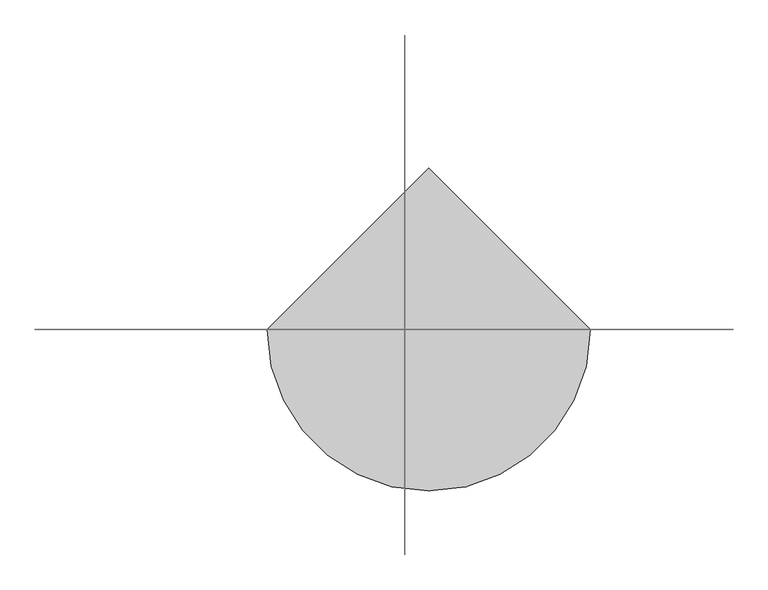
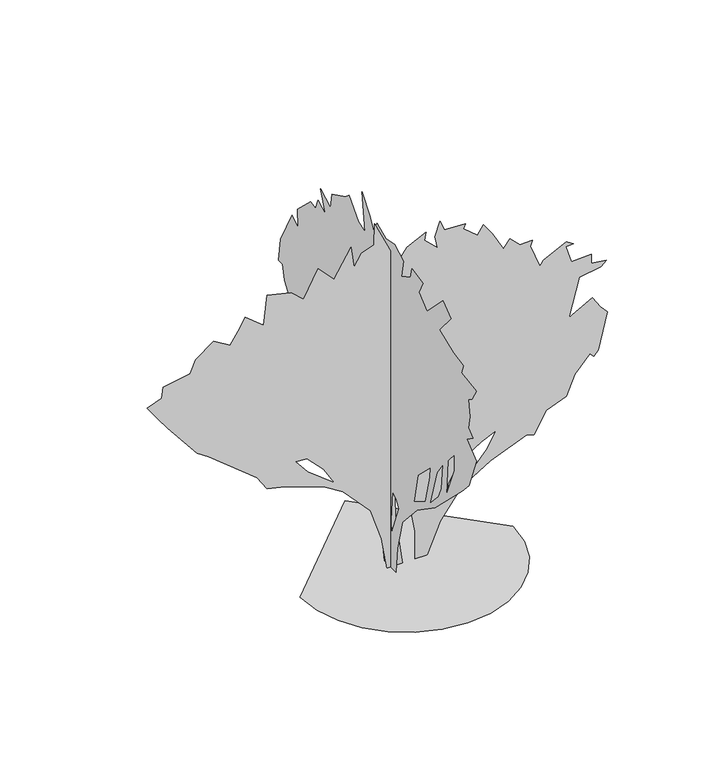
"""IFC4 building model written with IfcOpenShell, lengths in millimetres: proxy geometry, honey myrtle 26117 : honey myrtle 26117."""

from ifc_helpers import new_model, si_unit, origin, place, context, project, spatial, triangles, source, transform, mapped, element, save


def entourage_6475341c(model_context):
    return source(origin(), model_context, "Body", "Tessellation", [
        triangles([(-396.3767504, 0.0, 8.22e-05), (-385.8992649, -90.8237077, 8.22e-05), (-356.0543206, -174.2306261, 8.22e-05), (-309.2370838, -247.8313661, 8.22e-05), (-247.8313661, -309.2370838, 8.22e-05), (-174.2306261, -356.0543206, 8.22e-05), (-90.8237077, -385.8992649, 8.22e-05), (1.73e-05, -396.3767504, 8.22e-05), (90.8237077, -385.8992649, 8.22e-05), (174.2306261, -356.0543206, 8.22e-05), (247.8313661, -309.2370838, 8.22e-05), (309.2370838, -247.8313661, 8.22e-05), (356.0543206, -174.2306261, 8.22e-05), (385.8992649, -90.8237077, 8.22e-05), (396.3767504, 3.47e-05, 8.22e-05), (-5.2e-05, 396.3767504, 8.22e-05), (-59.3577095, -35.0059915, 9.26e-05), (-59.3577095, -44.8705806, 101.5460546), (-59.3577095, -75.4742449, 222.0478563), (-59.3577095, -168.9964434, 326.3007588), (-59.3577095, -285.8741748, 405.6706235), (-59.3579639, -459.2340692, 576.3228888), (-59.3579639, -503.9253456, 625.6344137), (-59.3579639, -553.1479589, 751.1941189), (-59.3579639, -491.6190474, 799.7715317), (-59.3579639, -530.478485, 828.915465), (-59.3579639, -501.3320083, 851.5849388), (-59.3579639, -511.0474763, 900.1598808), (-59.3579639, -501.3320083, 961.688756), (-59.3579639, -524.0014821, 977.8812269), (-59.3579639, -553.1479589, 1026.4561689), (-59.3579639, -455.9955677, 1039.4101748), (-59.3579639, -469.4956884, 1077.0376745), (-59.3579639, -404.1821606, 1087.9850441), (-59.3579639, -313.5068087, 1123.6085238), (-59.3579639, -387.9896896, 1211.0454105), (-59.3579639, -336.1762825, 1249.9048119), (-59.3579639, -235.7859349, 1149.5164627), (-59.3579639, -183.9712561, 1191.6144018), (-59.3579639, -209.8784683, 1243.4278816), (-59.3579639, -138.9198272, 1256.3183739), (-59.3579639, -128.9188388, 1217.5224134), (-59.3579639, -70.6279291, 1185.1373989), (-59.3579639, -83.5816624, 1253.143277), (-59.3579639, -25.4436618, 1284.1769932), (-59.3579639, 29.761912, 1272.5743584), (-59.3579639, 86.0073592, 1299.3586246), (-59.3579639, 110.7212849, 1256.3817421), (-59.3579639, 133.3899957, 1298.4822247), (-59.3579639, 185.2039207, 1363.2496376), (-59.3577095, 165.7739475, 1217.5224134), (-59.3577095, 207.8728858, 1230.4738758), (-59.3577095, 266.3644464, 1299.9199276), (-59.3577095, 292.0717617, 1279.0512886), (-59.3577095, 376.2676217, 1236.950806), (-59.3577095, 385.9830897, 1178.660396), (-59.3577095, 450.7505027, 1214.2838757), (-59.3577095, 418.3680679, 1133.3239918), (-59.3577095, 466.9429736, 1159.22946), (-59.3577095, 484.2835213, 1117.1086298), (-59.3577095, 515.5204227, 1123.6085238), (-59.3577095, 599.7162646, 1042.6486399), (-59.3577095, 596.4777632, 974.6427618), (-59.3577095, 635.3397079, 997.3122356), (-59.3577095, 709.8225889, 858.0619417), (-59.3577095, 722.7765947, 767.3865898), (-59.3577095, 696.8686558, 767.3865898), (-59.3577095, 683.91465, 712.3346449), (-59.3577095, 619.147237, 621.659293), (-59.3577095, 586.7622588, 628.1362959), (-59.3577095, 577.0493342, 595.7513177), (-59.3577095, 544.664356, 589.2743148), (-59.3577095, 512.2819213, 514.7914338), (-59.3577095, 453.9890041, 501.8400078), (-59.3577095, 473.4199765, 479.1705339), (-59.3577095, 438.083507, 433.2245012), (-59.3577095, 424.8450708, 430.5955919), (-59.3577095, 359.671251, 388.3935531), (-59.3577095, 230.5626891, 332.9860339), (-59.3577095, 112.6590482, 224.7923109), (-59.3577095, 55.1474106, 87.2636415), (-59.3577095, 39.476642, 8.38e-05), (-59.3577095, -5.8605105, 135.9018064), (-59.3577095, -2.7896791, 186.1833303), (-59.3577095, -12.337225, 304.2967785), (-59.3577095, -38.2442317, 288.1068329), (-59.3577095, -54.4362076, 262.1988576), (-59.3577095, -151.5875587, 349.6357444), (-59.3577095, -177.4947618, 469.4550296), (-59.3577095, -258.4549001, 547.176412), (-59.3577095, -255.2163986, 508.3169744), (-59.3577095, -226.0704487, 394.9721486), (-59.3577095, -255.2163986, 404.687653), (-59.3577095, -297.3143196, 550.4149135), (-59.3577095, -337.517407, 606.5056758), (-59.3577095, -326.4607781, 505.0785092), (-59.3577095, -307.0298058, 462.9780267), (-59.3577095, -358.8432129, 501.8400078), (-59.3579639, -368.5587173, 641.0903017), (-59.3579639, -410.6591635, 689.6651711), (-59.3579639, -410.6591635, 628.1362959), (-59.3577095, 198.157654, 356.112711), (-59.3577095, 261.769596, 391.7057055), (-59.3577095, 324.4541782, 475.9320325), (-59.3577095, 282.3562755, 469.4550296), (-59.3577095, 253.2100531, 430.5955919), (-267.2940953, 2.61e-05, 404.687653), (-308.6096875, 2.21e-05, 471.3142911), (-370.9208914, 1.84e-05, 534.2224425), (-413.0213739, 1.82e-05, 537.4609076), (-368.4215527, 2.15e-05, 482.1804156), (30.6369404, 5.02e-05, 0.0), (31.1304627, 4.38e-05, 108.1619844), (9.0696959, 3.61e-05, 237.4841779), (-47.0839311, 3.05e-05, 330.2047357), (-39.4309189, 4.01e-05, 170.4041154), (-14.7000316, 5.02e-05, 0.0), (-72.990889, 5.02e-05, 0.0), (-92.9872747, 4.29e-05, 122.5858678), (-134.4006626, 3.55e-05, 247.1552083), (-236.0793036, 2.88e-05, 358.7517941), (-302.2063538, 2.64e-05, 398.8659516), (-451.8807753, 2.32e-05, 453.2625587), (-519.8892331, 2.22e-05, 469.4550296), (-555.510133, 1.89e-05, 524.5069382), (-736.858366, 1.03e-05, 670.234235), (-778.9587759, 8.5e-06, 699.3807117), (-889.0625931, 4e-07, 835.3924679), (-924.6860727, -2.5e-06, 883.9674099), (-965.6003632, -6e-06, 942.4685629), (-911.7320669, -7.1e-06, 961.688756), (-905.255064, -9.6e-06, 1003.7892385), (-804.8642441, -1.06e-05, 1019.979166), (-785.4357788, -1.35e-05, 1068.5565788), (-717.4299007, -1.64e-05, 1117.1315208), (-655.8984821, -1.43e-05, 1081.5105846), (-620.2775459, -1.75e-05, 1136.5625296), (-600.8465735, -1.97e-05, 1172.1833931), (-532.8406591, -1.64e-05, 1117.1315208), (-519.8892331, -2.31e-05, 1230.4738758), (-429.2138449, -2.18e-05, 1207.8068727), (-383.8748972, -1.93e-05, 1165.7064629), (-328.8229886, -2.53e-05, 1266.0972828), (-270.5325967, -2.16e-05, 1204.5684076), (-205.7644389, -2.78e-05, 1308.1951492), (-196.0496976, -2.29e-05, 1227.2378815), (-167.6639666, -2.55e-05, 1270.8241745), (-121.5665623, -2.66e-05, 1288.7668293), (-119.7654549, -3.15e-05, 1371.5986919), (-34.1304544, -2.06e-05, 1188.3759367), (2.3015577, -2.34e-05, 1235.4267712), (72.7363851, -2.54e-05, 1269.3357479), (66.2596456, -2.37e-05, 1240.1892712), (114.8353143, -2.1e-05, 1194.8529396), (105.1200825, -2.37e-05, 1240.1892712), (124.5505553, -2.7e-05, 1295.2437595), (140.7425266, -2.47e-05, 1256.3817421), (218.4636638, -2.45e-05, 1253.143277), (211.1367854, -2.35e-05, 1235.7950626), (263.8015941, -2.08e-05, 1191.6144018), (286.4685245, -2.27e-05, 1223.9994164), (318.8535027, -2e-05, 1178.660396), (360.9514054, -1.56e-05, 1104.177515), (385.0814006, -1.75e-05, 1135.7446289), (422.4828604, -1.52e-05, 1097.7005121), (467.8192646, -1.54e-05, 1100.9390499), (461.3422617, -1.41e-05, 1078.2721195), (496.9657413, -8.7e-06, 987.5967676), (509.9172037, -9.8e-06, 1007.0277037), (594.1155527, -1.23e-05, 1049.1256428), (620.0235643, -1.14e-05, 1032.9331718), (593.290058, -1.13e-05, 1031.1069025), (613.5465614, -7.3e-06, 964.9272211), (688.0294424, -7.5e-06, 968.1657589), (688.0294424, -5.4e-06, 932.5448227), (743.0813147, -5e-06, 926.0678198), (723.6503786, -3.8e-06, 906.6368837), (642.6904947, -3.1e-06, 893.6828779), (603.8310571, 5.6e-06, 747.9555811), (691.2679075, 2.7e-06, 796.5330666), (720.4118408, 5.4e-06, 751.1941189), (746.3198524, 7.2e-06, 722.0501856), (713.9348379, 1.55e-05, 582.7973482), (697.7449104, 1.66e-05, 563.3688829), (681.5524395, 1.57e-05, 579.5613902), (626.5005672, 1.93e-05, 518.0299353), (594.1155527, 2.38e-05, 443.5470543), (519.6326717, 2.55e-05, 414.403121), (474.2962675, 3.03e-05, 333.4432371), (448.3882922, 2.98e-05, 343.1587415), (311.7719945, 3.3e-05, 288.0331637), (205.1723602, 3.7e-05, 221.2502851), (125.3034072, 4.32e-05, 117.1220752), (75.9746277, 5.02e-05, 0.0), (30.6369404, 3.34e-05, 281.62983), (43.5909303, 2.72e-05, 385.2566442), (7.9686832, 2.28e-05, 459.7395252), (-30.8919575, 2.45e-05, 430.5955919), (-38.6976243, 2.72e-05, 386.112624), (-2.6646859, 3.14e-05, 315.8842435), (150.4575132, 3.75e-05, 213.6229345), (215.0437962, 3.57e-05, 242.9182394), (296.5269221, 3.01e-05, 337.5199505), (331.8074721, 2.65e-05, 398.2106501), (278.0814637, 2.79e-05, 375.0661689), (195.3344433, 3.11e-05, 320.3901821), (154.7673882, 3.52e-05, 251.8887493)], [[15, 16, 1], [14, 15, 1], [14, 1, 2], [13, 14, 2], [13, 2, 3], [13, 3, 4], [12, 13, 4], [11, 12, 4], [11, 4, 5], [11, 5, 6], [11, 6, 7], [11, 7, 8], [11, 8, 9], [11, 9, 10], [93, 90, 91], [93, 91, 92], [90, 93, 94], [95, 98, 99], [83, 17, 18], [98, 95, 96], [49, 50, 51], [56, 57, 58], [88, 85, 86], [48, 49, 51], [102, 84, 85], [83, 18, 19], [87, 83, 19], [30, 31, 32], [87, 19, 20], [39, 40, 41], [39, 41, 42], [25, 26, 27], [29, 30, 32], [82, 17, 83], [81, 82, 83], [80, 81, 83], [80, 83, 84], [80, 84, 102], [79, 80, 102], [79, 102, 103], [78, 79, 103], [78, 103, 104], [77, 78, 104], [32, 33, 34], [65, 66, 67], [58, 59, 60], [35, 36, 37], [35, 37, 38], [88, 86, 87], [88, 87, 20], [92, 88, 20], [92, 20, 21], [93, 92, 21], [97, 93, 21], [97, 21, 22], [63, 64, 65], [52, 53, 54], [46, 47, 48], [74, 75, 76], [23, 24, 25], [43, 44, 45], [43, 45, 46], [98, 96, 97], [98, 97, 22], [101, 98, 22], [101, 22, 23], [101, 23, 25], [100, 101, 25], [68, 69, 70], [74, 76, 77], [74, 77, 104], [70, 71, 72], [85, 88, 89], [102, 85, 89], [106, 102, 89], [105, 106, 89], [52, 54, 55], [52, 55, 56], [60, 61, 62], [60, 62, 63], [39, 42, 43], [72, 73, 74], [43, 46, 48], [43, 48, 51], [63, 65, 67], [90, 94, 95], [105, 89, 90], [38, 39, 43], [63, 67, 68], [63, 68, 70], [63, 70, 72], [60, 63, 72], [58, 60, 72], [58, 72, 74], [58, 74, 104], [58, 104, 105], [58, 105, 90], [56, 58, 90], [52, 56, 90], [51, 52, 90], [43, 51, 90], [38, 43, 90], [38, 90, 95], [38, 95, 99], [38, 99, 100], [35, 38, 100], [35, 100, 25], [35, 25, 27], [34, 35, 27], [32, 34, 27], [29, 32, 27], [28, 29, 27], [196, 112, 113], [196, 197, 201], [195, 196, 113], [195, 113, 114], [148, 149, 150], [112, 196, 201], [170, 171, 172], [207, 201, 197], [144, 145, 146], [155, 156, 157], [175, 176, 177], [175, 177, 178], [151, 152, 153], [194, 112, 201], [193, 194, 201], [192, 193, 201], [192, 201, 202], [191, 192, 202], [191, 202, 203], [195, 114, 115], [200, 195, 115], [199, 200, 115], [169, 170, 172], [206, 207, 197], [157, 158, 159], [165, 166, 167], [160, 161, 162], [142, 143, 144], [129, 130, 131], [116, 117, 118], [116, 118, 119], [116, 119, 120], [115, 116, 120], [107, 115, 120], [107, 120, 121], [107, 121, 122], [111, 107, 122], [111, 122, 123], [110, 111, 123], [137, 138, 139], [199, 115, 107], [163, 164, 165], [139, 140, 141], [183, 184, 185], [190, 191, 203], [190, 203, 204], [173, 174, 175], [173, 175, 178], [169, 172, 173], [179, 180, 181], [198, 199, 107], [139, 141, 142], [188, 189, 190], [110, 123, 124], [110, 124, 125], [168, 169, 173], [154, 155, 157], [154, 157, 159], [131, 132, 133], [182, 183, 185], [188, 190, 204], [147, 148, 150], [146, 147, 150], [205, 206, 197], [136, 137, 139], [181, 182, 185], [179, 181, 185], [179, 185, 186], [134, 135, 136], [198, 107, 108], [154, 159, 160], [133, 134, 136], [168, 173, 178], [168, 178, 179], [129, 131, 133], [128, 129, 133], [127, 128, 133], [127, 133, 136], [126, 127, 136], [126, 136, 139], [125, 126, 139], [110, 125, 139], [110, 139, 142], [109, 110, 142], [109, 142, 144], [109, 144, 146], [109, 146, 150], [108, 109, 150], [198, 108, 150], [197, 198, 150], [205, 197, 150], [204, 205, 150], [188, 204, 150], [187, 188, 150], [186, 187, 150], [179, 186, 150], [168, 179, 150], [167, 168, 150], [150, 151, 153], [150, 153, 154], [160, 162, 163], [154, 160, 163], [150, 154, 163], [167, 150, 163], [167, 163, 165]], closed=False),
    ])


if __name__ == "__main__":
    model = new_model("IFC4")
    model_context = context("Model", 3, world=origin())
    ifc_project = project(units=[si_unit("LENGTHUNIT", "METRE", prefix="MILLI")], contexts=[model_context])
    site = spatial("IfcSite", under=ifc_project)
    building = spatial("IfcBuilding", under=site)
    placement = place(None, origin())
    entourage_shape = entourage_6475341c(model_context)
    element("IfcBuildingElementProxy", 1, Name="honey myrtle 26117 : honey myrtle 26117", ObjectType="honey myrtle 26117 : honey myrtle 26117", at=placement, inside=building, context=model_context, shape_type="MappedRepresentation", body=[
        mapped(entourage_shape, transform((0.0, 0.0, 0.0), x_axis=(1.0, 0.0, 0.0), y_axis=(0.0, 1.0, 0.0), z_axis=(0.0, 0.0, 1.0))),
    ])
    save(model, "model.ifc")

# Revit data of these elements
# Type "honey myrtle 26117 : honey myrtle 26117"
#   built-in parameter 1005195 = "RPC-16-G3GK-N2Q0-PN0G-6000-ST1L-LVER-AU"
#   Height = 0
